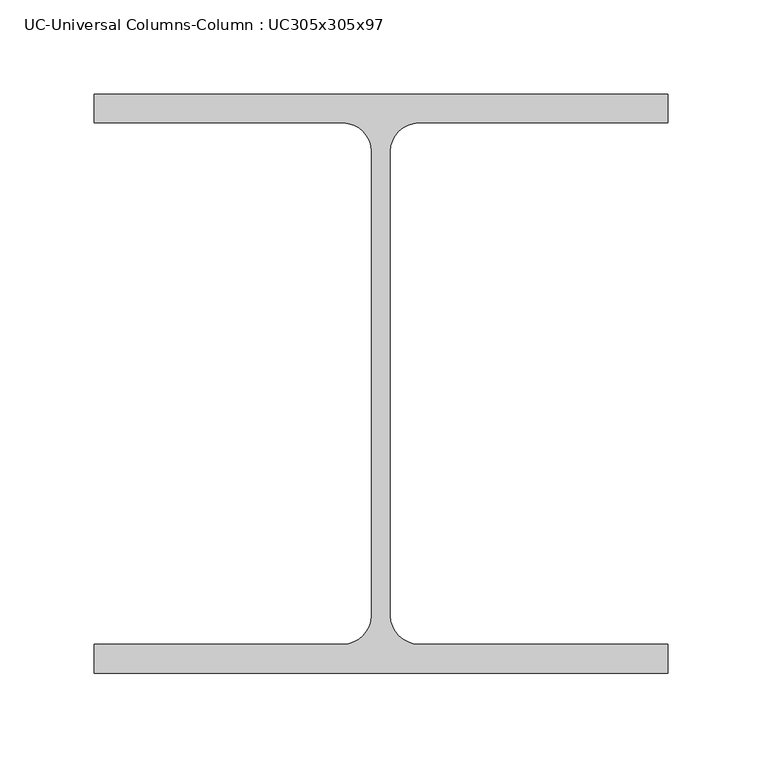
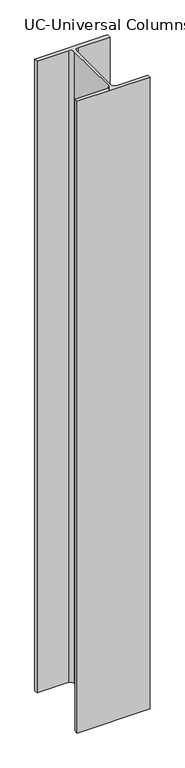
"""IFC4 building model written with IfcOpenShell, lengths in millimetres: column geometry, UC-Universal Columns-Column : UC305x305x97."""

import ifcopenshell
import ifcopenshell.guid

model = None  # the IFC model being written
_history = None  # IfcOwnerHistory: only IFC2X3 demands one
_inside = {}  # id of a spatial element -> (the spatial element, [elements in it])
_under = {}  # id of a project, library or spatial element -> (it, [spatial elements below it])
_declared = {}  # id of a project -> (the project, [libraries it declares])
_typed = {}  # id of a type object -> (the type object, [elements of that type])
_made_of = {}  # id of a material, layer set ... -> (it, [elements and type objects made of it])


def new_model(schema):
    """Start an empty IFC model of exactly this schema.

    Asked for "IFC4X3", IfcOpenShell would pick the latest addendum, in which some entities
    have other attributes; the version numbers below select the first issue.
    IFC2X3 requires an IfcOwnerHistory on every rooted entity: one is made here for all.
    """
    global model, _history
    if schema == "IFC4X3":
        model = ifcopenshell.file(schema_version=(4, 3, 0, 0))
    else:
        model = ifcopenshell.file(schema=schema)
    _inside.clear()
    _under.clear()
    _declared.clear()
    _typed.clear()
    _made_of.clear()
    _history = None
    if model.schema == "IFC2X3":
        org = make("IfcOrganization", Name="unknown")
        user = make(
            "IfcPersonAndOrganization",
            ThePerson=make("IfcPerson", FamilyName="unknown"),
            TheOrganization=org,
        )
        app = make(
            "IfcApplication",
            ApplicationDeveloper=org,
            Version="unknown",
            ApplicationFullName="unknown",
            ApplicationIdentifier="unknown",
        )
        _history = make(
            "IfcOwnerHistory",
            OwningUser=user,
            OwningApplication=app,
            ChangeAction="ADDED",
            CreationDate=0,
        )
    return model


def make(cls, **values):
    """One entity of the class cls with the attributes given. An attribute that is None is left unset."""
    return model.create_entity(
        cls, **{name: value for name, value in values.items() if value is not None}
    )


def rooted(cls, **values):
    """An entity with a GlobalId (a new one), such as an element, a storey or a relation."""
    return make(cls, GlobalId=ifcopenshell.guid.new(), OwnerHistory=_history, **values)


def si_unit(unit_type, name, prefix=None):
    """IfcSIUnit, for example si_unit("LENGTHUNIT", "METRE", prefix="MILLI")."""
    return make("IfcSIUnit", UnitType=unit_type, Prefix=prefix, Name=name)


def assignment(units):
    """IfcUnitAssignment: the units of a project."""
    return None if units is None else make("IfcUnitAssignment", Units=units)


def point(xyz):
    """IfcCartesianPoint."""
    return None if xyz is None else make("IfcCartesianPoint", Coordinates=xyz)


def direction(xyz):
    """IfcDirection."""
    return None if xyz is None else make("IfcDirection", DirectionRatios=xyz)


def frame(location, z_axis=None, x_axis=None):
    """IfcAxis2Placement3D, a coordinate frame: its origin and axes. An axis left out is left unset."""
    return make(
        "IfcAxis2Placement3D",
        Location=point(location),
        Axis=direction(z_axis),
        RefDirection=direction(x_axis),
    )


def frame_2d(location, x_axis=None):
    """IfcAxis2Placement2D, a coordinate frame in the plane: its origin and x axis."""
    return make(
        "IfcAxis2Placement2D", Location=point(location), RefDirection=direction(x_axis)
    )


def origin():
    """The frame at (0, 0, 0) with its axes left unset."""
    return frame((0.0, 0.0, 0.0))


def place(relative_to, where):
    """IfcLocalPlacement: puts the frame where relative to a parent placement (None: the world)."""
    return make(
        "IfcLocalPlacement", PlacementRelTo=relative_to, RelativePlacement=where
    )


def context(
    kind, dimensions, precision=None, world=None, true_north=None, identifier=None
):
    """IfcGeometricRepresentationContext, for example the 3D "Model" context."""
    return make(
        "IfcGeometricRepresentationContext",
        ContextIdentifier=identifier,
        ContextType=kind,
        CoordinateSpaceDimension=dimensions,
        Precision=precision,
        WorldCoordinateSystem=world,
        TrueNorth=true_north,
    )


def project(units=None, contexts=None):
    """IfcProject with its units and contexts."""
    return rooted(
        "IfcProject",
        Name="project",
        RepresentationContexts=contexts,
        UnitsInContext=assignment(units),
    )


def spatial(cls, under=None, at=None, **own):
    """A site, building, storey or space (cls), placed at a placement, below another one or the project."""
    s = rooted(cls, ObjectPlacement=at, **own)
    if under is not None:
        _under.setdefault(under.id(), (under, []))[1].append(s)
    return s


def polyline(points):
    """IfcPolyline through the points."""
    return make("IfcPolyline", Points=[point(p) for p in points])


def circle_curve(where, radius):
    """IfcCircle in the frame where."""
    return make("IfcCircle", Position=where, Radius=radius)


def trimmed(basis, trim1, trim2, sense, master):
    """IfcTrimmedCurve: the piece of a basis curve between two trims."""
    return make(
        "IfcTrimmedCurve",
        BasisCurve=basis,
        Trim1=trim1,
        Trim2=trim2,
        SenseAgreement=sense,
        MasterRepresentation=master,
    )


def segment(curve, same_sense, transition):
    """IfcCompositeCurveSegment."""
    return make(
        "IfcCompositeCurveSegment",
        Transition=transition,
        SameSense=same_sense,
        ParentCurve=curve,
    )


def composite_curve(segments, self_intersect=None):
    """IfcCompositeCurve: segments joined end to end."""
    return make("IfcCompositeCurve", Segments=segments, SelfIntersect=self_intersect)


def outline(outer, holes=None, kind="AREA"):
    """IfcArbitraryClosedProfileDef: a profile drawn as a closed curve; with holes, ...WithVoids."""
    if holes is None:
        return make("IfcArbitraryClosedProfileDef", ProfileType=kind, OuterCurve=outer)
    return make(
        "IfcArbitraryProfileDefWithVoids",
        ProfileType=kind,
        OuterCurve=outer,
        InnerCurves=holes,
    )


def extrude(swept, where, along, depth):
    """IfcExtrudedAreaSolid: the profile swept, set in the frame where, extruded along a direction by depth."""
    return make(
        "IfcExtrudedAreaSolid",
        SweptArea=swept,
        Position=where,
        ExtrudedDirection=direction(along),
        Depth=depth,
    )


def shape(context_of_items, identifier, shape_type, items):
    """IfcShapeRepresentation: the items that make up one representation, for example the "Body"."""
    return make(
        "IfcShapeRepresentation",
        ContextOfItems=context_of_items,
        RepresentationIdentifier=identifier,
        RepresentationType=shape_type,
        Items=items,
    )


def source(mapping_origin, context_of_items, identifier, shape_type, items):
    """IfcRepresentationMap: a shape defined once, which mapped items show again and again."""
    return make(
        "IfcRepresentationMap",
        MappingOrigin=mapping_origin,
        MappedRepresentation=shape(context_of_items, identifier, shape_type, items),
    )


def transform(
    local_origin,
    x_axis=None,
    y_axis=None,
    z_axis=None,
    scale=None,
    scale2=None,
    scale3=None,
    uniform=True,
):
    """IfcCartesianTransformationOperator3D, or its non-uniform kind. x_axis, y_axis, z_axis: its Axis1, 2, 3."""
    if uniform:
        return make(
            "IfcCartesianTransformationOperator3D",
            Axis1=direction(x_axis),
            Axis2=direction(y_axis),
            LocalOrigin=point(local_origin),
            Scale=scale,
            Axis3=direction(z_axis),
        )
    return make(
        "IfcCartesianTransformationOperator3DnonUniform",
        Axis1=direction(x_axis),
        Axis2=direction(y_axis),
        LocalOrigin=point(local_origin),
        Scale=scale,
        Axis3=direction(z_axis),
        Scale2=scale2,
        Scale3=scale3,
    )


def mapped(mapping_source, mapping_target):
    """IfcMappedItem: shows the shape of a source again, moved by a transform."""
    return make(
        "IfcMappedItem", MappingSource=mapping_source, MappingTarget=mapping_target
    )


def made_of(thing, what):
    """Note that an element or type object is made of a material, layer set ...; save() writes the relation."""
    if what is not None:
        _made_of.setdefault(what.id(), (what, []))[1].append(thing)
    return thing


def element(
    cls,
    number,
    at=None,
    inside=None,
    cuts=None,
    type_object=None,
    material=None,
    context=None,
    identifier="Body",
    shape_type=None,
    held_by="IfcProductDefinitionShape",
    body=None,
    shapes=None,
    **own,
):
    """One element of the class cls, such as IfcWall. Its Tag is "e" and its number.

    at: its placement. inside: the storey or other place that contains it. cuts: it is an
    opening in that element (IfcRelVoidsElement). A single representation is given by context,
    identifier, shape_type and body (its items); several are given by shapes. held_by: the class
    of the entity that holds the representations. save() writes the other relations.
    """
    e = rooted(cls, Tag="e%d" % number, ObjectPlacement=at, **own)
    if body is not None:
        shapes = [shape(context, identifier, shape_type, body)]
    if shapes is not None:
        e.Representation = make(held_by, Representations=shapes)
    if inside is not None:
        _inside.setdefault(inside.id(), (inside, []))[1].append(e)
    if cuts is not None:
        rooted(
            "IfcRelVoidsElement", RelatingBuildingElement=cuts, RelatedOpeningElement=e
        )
    if type_object is not None:
        _typed.setdefault(type_object.id(), (type_object, []))[1].append(e)
    return made_of(e, material)


def aggregate(whole, parts):
    """IfcRelAggregates: a whole, such as a stair, and the parts it consists of."""
    return rooted("IfcRelAggregates", RelatingObject=whole, RelatedObjects=parts)


def save(model, path):
    """Write the relations noted so far, then the file.

    IfcRelAggregates (storeys below a building ...), IfcRelContainedInSpatialStructure (elements
    in a storey), IfcRelDefinesByType, IfcRelAssociatesMaterial and IfcRelDeclares: one each for
    every whole, place, type object, material and project.
    """
    for whole, parts in _under.values():
        aggregate(whole, parts)
    for where, things in _inside.values():
        rooted(
            "IfcRelContainedInSpatialStructure",
            RelatedElements=things,
            RelatingStructure=where,
        )
    for kind, things in _typed.values():
        rooted("IfcRelDefinesByType", RelatedObjects=things, RelatingType=kind)
    for what, things in _made_of.values():
        rooted("IfcRelAssociatesMaterial", RelatedObjects=things, RelatingMaterial=what)
    for by, libraries in _declared.values():
        rooted("IfcRelDeclares", RelatingContext=by, RelatedDefinitions=libraries)
    model.write(path)


def uc_universal_columns_column_uc305x305x97_6ea2ceb4(model_context):
    return source(origin(), model_context, "Body", "SweptSolid", [
        extrude(outline(composite_curve([segment(polyline([(152.65, 153.95), (152.65, 138.55), (20.15, 138.55)]), True, "CONTINUOUS"), segment(trimmed(circle_curve(frame_2d((20.15, 123.35)), 15.2), [point((20.15, 138.55))], [point((4.95, 123.35))], True, "CARTESIAN"), True, "CONTINUOUS"), segment(polyline([(4.95, 123.35), (4.95, -123.35)]), True, "CONTINUOUS"), segment(trimmed(circle_curve(frame_2d((20.15, -123.35)), 15.2), [point((4.95, -123.35))], [point((20.15, -138.55))], True, "CARTESIAN"), True, "CONTINUOUS"), segment(polyline([(20.15, -138.55), (152.65, -138.55), (152.65, -153.95), (-152.65, -153.95), (-152.65, -138.55), (-20.15, -138.55)]), True, "CONTINUOUS"), segment(trimmed(circle_curve(frame_2d((-20.15, -123.35)), 15.2), [point((-20.15, -138.55))], [point((-4.95, -123.35))], True, "CARTESIAN"), True, "CONTINUOUS"), segment(polyline([(-4.95, -123.35), (-4.95, 123.35)]), True, "CONTINUOUS"), segment(trimmed(circle_curve(frame_2d((-20.15, 123.35)), 15.2), [point((-4.95, 123.35))], [point((-20.15, 138.55))], True, "CARTESIAN"), True, "CONTINUOUS"), segment(polyline([(-20.15, 138.55), (-152.65, 138.55), (-152.65, 153.95), (152.65, 153.95)]), True, "CONTINUOUS")], self_intersect=False)), frame((0.0, 0.0, -594.0), z_axis=(0.0, 0.0, 1.0), x_axis=(1.0, 0.0, 0.0)), (0.0, 0.0, 1.0), 2793.0),
    ])


if __name__ == "__main__":
    model = new_model("IFC4")
    model_context = context("Model", 3, world=origin())
    ifc_project = project(units=[si_unit("LENGTHUNIT", "METRE", prefix="MILLI")], contexts=[model_context])
    site = spatial("IfcSite", under=ifc_project)
    building = spatial("IfcBuilding", under=site)
    placement = place(None, origin())
    uc_universal_columns_column_uc305x305x97_shape = uc_universal_columns_column_uc305x305x97_6ea2ceb4(model_context)
    element("IfcColumn", 1, ObjectType="UC-Universal Columns-Column : UC305x305x97", at=placement, inside=building, context=model_context, shape_type="MappedRepresentation", body=[
        mapped(uc_universal_columns_column_uc305x305x97_shape, transform((0.0, 0.0, 0.0), x_axis=(1.0, 0.0, 0.0), y_axis=(0.0, 1.0, 0.0), z_axis=(0.0, 0.0, 1.0))),
    ])
    save(model, "model.ifc")

# Revit data of these elements
# Type "UC-Universal Columns-Column : UC305x305x97"
#   Section Name Key = "UC305x305x97"
#   Cost = 5
#   Width = 30.53 cm
#   Web Thickness = 0.99 cm
#   Web Fillet = 1.52 cm
#   Warping Constant = 1560000.0 cm⁶
#   Torsional Moment of Inertia = 91.20 cm⁴
#   Section Area = 123.0 cm²
#   Plastic Modulus weak axis = 726.0 cm³
#   Plastic Modulus strong axis = 1592.0 cm³
#   Nominal Weight = 96.8996 kgf/m
#   Moment of Inertia weak axis = 7308.00 cm⁴
#   Moment of Inertia strong axis = 22249.00 cm⁴
#   Height = 30.79 cm
#   Flange Thickness = 1.54 cm
#   Elastic Modulus weak axis = 479.0 cm³
#   Elastic Modulus strong axis = 1445.0 cm³
#   Centroid Vertical = 15.395 cm
#   Centroid Horizontal = 15.265 cm
#   Bolt Spacing = 14.0 cm
#   Structural Material [instance default] = Metal - Steel 43-275
#   Type Comments = ""
#   Assembly Code = ""
# Element 1 (IfcColumn, "UC-Universal Columns-Column : UC305x305x97")
#   Materials on its faces: "Metal - Steel 43-275"
# Materials
#   "Metal - Steel 43-275": class "Metal", colour RGB 247 247 247, transparency 0, Cost = 0
